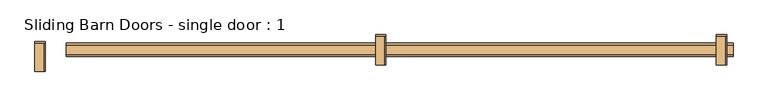
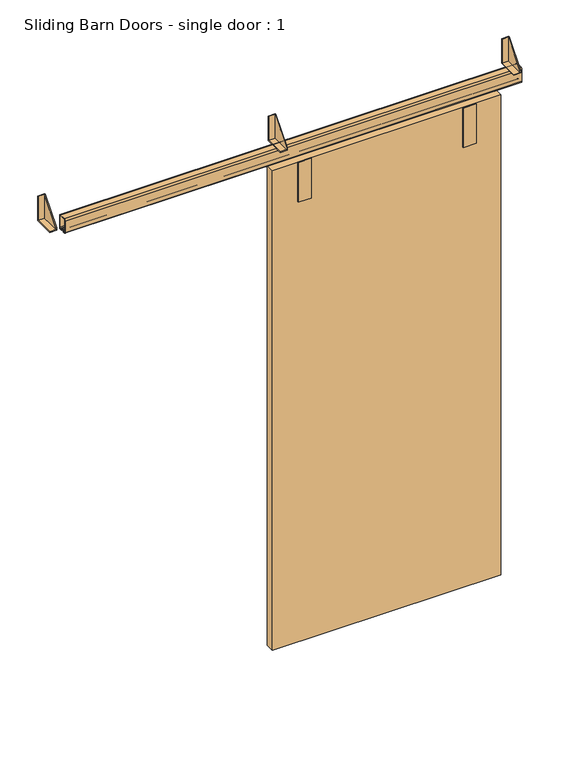
"""IFC4 building model written with IfcOpenShell, lengths in millimetres: door geometry, Sliding Barn Doors - single door : 1."""

from ifc_helpers import new_model, si_unit, point, frame, frame_2d, origin, place, context, project, spatial, polyline, circle_curve, trimmed, segment, composite_curve, outline, extrude, source, transform, mapped, element, save


def sliding_barn_doors_single_door_1_9618ed7f(model_context):
    return source(origin(), model_context, "Body", "SweptSolid", [
        extrude(outline(polyline([(-158.75, 2152.65), (-79.375, 2247.773), (-79.375, 2146.3), (-158.75, 2146.3), (-158.75, 2152.65)])), frame((-1418.4808594, 0.0, 0.0), z_axis=(1.0, 0.0, 0.0), x_axis=(0.0, 1.0, 0.0)), (0.0, 0.0, 1.0), 3.175),
        extrude(outline(polyline([(-76.2, 2143.125), (-158.75, 2143.125), (-158.75, 2146.3), (-79.375, 2146.3), (-79.375, 2247.773), (-76.2, 2247.773), (-76.2, 2143.125)])), frame((-1443.7816406, 0.0, 0.0), z_axis=(1.0, 0.0, 0.0), x_axis=(0.0, 1.0, 0.0)), (0.0, 0.0, 1.0), 28.4757812),
        extrude(outline(polyline([(-139.7, 2152.65), (-60.325, 2247.773), (-60.325, 2146.3), (-139.7, 2146.3), (-139.7, 2152.65)])), frame((-484.2371094, 0.0, 0.0), z_axis=(1.0, 0.0, 0.0), x_axis=(0.0, 1.0, 0.0)), (0.0, 0.0, 1.0), 3.175),
        extrude(outline(polyline([(-57.15, 2143.125), (-139.7, 2143.125), (-139.7, 2146.3), (-60.325, 2146.3), (-60.325, 2247.773), (-57.15, 2247.773), (-57.15, 2143.125)])), frame((-509.5378906, 0.0, 0.0), z_axis=(1.0, 0.0, 0.0), x_axis=(0.0, 1.0, 0.0)), (0.0, 0.0, 1.0), 28.4757813),
        extrude(outline(polyline([(-139.7, 2152.65), (-60.325, 2247.773), (-60.325, 2146.3), (-139.7, 2146.3), (-139.7, 2152.65)])), frame((450.0066406, 0.0, 0.0), z_axis=(1.0, 0.0, 0.0), x_axis=(0.0, 1.0, 0.0)), (0.0, 0.0, 1.0), 3.175),
        extrude(outline(polyline([(-57.15, 2143.125), (-139.7, 2143.125), (-139.7, 2146.3), (-60.325, 2146.3), (-60.325, 2247.773), (-57.15, 2247.773), (-57.15, 2143.125)])), frame((424.7058594, 0.0, 0.0), z_axis=(1.0, 0.0, 0.0), x_axis=(0.0, 1.0, 0.0)), (0.0, 0.0, 1.0), 28.4757813),
        extrude(outline(polyline([(-424.91025, -117.475), (-424.91025, -114.3), (-373.60225, -114.3), (-373.60225, -117.475), (-424.91025, -117.475)])), frame((0.0, 0.0, 1889.252), z_axis=(0.0, 0.0, 1.0), x_axis=(1.0, 0.0, 0.0)), (0.0, 0.0, 1.0), 168.148),
        extrude(outline(polyline([(235.48975, -117.475), (235.48975, -114.3), (286.79775, -114.3), (286.79775, -117.475), (235.48975, -117.475)])), frame((0.0, 0.0, 1889.252), z_axis=(0.0, 0.0, 1.0), x_axis=(1.0, 0.0, 0.0)), (0.0, 0.0, 1.0), 168.148),
        extrude(outline(polyline([(-526.25625, -114.3), (-526.25625, -79.375), (388.14375, -79.375), (388.14375, -114.3), (-526.25625, -114.3)])), frame((0.0, 0.0, 25.4), z_axis=(0.0, 0.0, 1.0), x_axis=(1.0, 0.0, 0.0)), (0.0, 0.0, 1.0), 2032.0),
        extrude(outline(composite_curve([segment(trimmed(circle_curve(frame_2d((-85.725, 2136.775)), 6.35), [point((-85.725, 2143.125))], [point((-79.375, 2136.775))], False, "CARTESIAN"), True, "CONTINUOUS"), segment(polyline([(-79.375, 2136.775), (-79.375, 2088.515)]), True, "CONTINUOUS"), segment(trimmed(circle_curve(frame_2d((-85.725, 2088.515)), 6.35), [point((-79.375, 2088.515))], [point((-85.725, 2082.165))], False, "CARTESIAN"), True, "CONTINUOUS"), segment(polyline([(-85.725, 2082.165), (-91.1336853, 2082.165)]), True, "CONTINUOUS"), segment(trimmed(circle_curve(frame_2d((-91.1336853, 2083.7525)), 1.5875), [point((-91.1336853, 2082.165))], [point((-92.6920184, 2083.4495907))], False, "CARTESIAN"), True, "CONTINUOUS"), segment(polyline([(-92.6920184, 2083.4495907), (-94.1175341, 2090.7832331), (-92.6013971, 2090.7832331), (-91.2154749, 2083.6532812), (-85.725, 2083.6532812)]), True, "CONTINUOUS"), segment(trimmed(circle_curve(frame_2d((-85.725, 2088.515)), 4.8617187), [point((-85.725, 2083.6532812))], [point((-80.8632813, 2088.515))], True, "CARTESIAN"), True, "CONTINUOUS"), segment(polyline([(-80.8632813, 2088.515), (-80.8632813, 2136.775)]), True, "CONTINUOUS"), segment(trimmed(circle_curve(frame_2d((-85.725, 2136.775)), 4.8617187), [point((-80.8632813, 2136.775))], [point((-85.725, 2141.6367187))], True, "CARTESIAN"), True, "CONTINUOUS"), segment(polyline([(-85.725, 2141.6367187), (-111.252, 2141.6367187)]), True, "CONTINUOUS"), segment(trimmed(circle_curve(frame_2d((-111.252, 2136.775)), 4.8617187), [point((-111.252, 2141.6367187))], [point((-116.1137188, 2136.775))], True, "CARTESIAN"), True, "CONTINUOUS"), segment(polyline([(-116.1137188, 2136.775), (-116.1137188, 2088.515)]), True, "CONTINUOUS"), segment(trimmed(circle_curve(frame_2d((-111.252, 2088.515)), 4.8617187), [point((-116.1137188, 2088.515))], [point((-111.252, 2083.6532812))], True, "CARTESIAN"), True, "CONTINUOUS"), segment(polyline([(-111.252, 2083.6532812), (-105.7615251, 2083.6532812), (-104.3756029, 2090.7832331), (-102.8594659, 2090.7832331), (-104.2849816, 2083.4495907)]), True, "CONTINUOUS"), segment(trimmed(circle_curve(frame_2d((-105.8433147, 2083.7525)), 1.5875), [point((-104.2849816, 2083.4495907))], [point((-105.8433147, 2082.165))], False, "CARTESIAN"), True, "CONTINUOUS"), segment(polyline([(-105.8433147, 2082.165), (-111.252, 2082.165)]), True, "CONTINUOUS"), segment(trimmed(circle_curve(frame_2d((-111.252, 2088.515)), 6.35), [point((-111.252, 2082.165))], [point((-117.602, 2088.515))], False, "CARTESIAN"), True, "CONTINUOUS"), segment(polyline([(-117.602, 2088.515), (-117.602, 2136.775)]), True, "CONTINUOUS"), segment(trimmed(circle_curve(frame_2d((-111.252, 2136.775)), 6.35), [point((-117.602, 2136.775))], [point((-111.252, 2143.125))], False, "CARTESIAN"), True, "CONTINUOUS"), segment(polyline([(-111.252, 2143.125), (-85.725, 2143.125)]), True, "CONTINUOUS")], self_intersect=False)), frame((-1358.10625, 0.0, 0.0), z_axis=(1.0, 0.0, 0.0), x_axis=(0.0, 1.0, 0.0)), (0.0, 0.0, 1.0), 1828.8),
    ])


if __name__ == "__main__":
    model = new_model("IFC4")
    model_context = context("Model", 3, world=origin())
    ifc_project = project(units=[si_unit("LENGTHUNIT", "METRE", prefix="MILLI")], contexts=[model_context])
    site = spatial("IfcSite", under=ifc_project)
    building = spatial("IfcBuilding", under=site)
    placement = place(None, origin())
    sliding_barn_doors_single_door_1_shape = sliding_barn_doors_single_door_1_9618ed7f(model_context)
    element("IfcDoor", 1, ObjectType="Sliding Barn Doors - single door : 1", at=placement, inside=building, context=model_context, shape_type="MappedRepresentation", body=[
        mapped(sliding_barn_doors_single_door_1_shape, transform((0.0, 0.0, 0.0), x_axis=(1.0, 0.0, 0.0), y_axis=(0.0, 1.0, 0.0), z_axis=(0.0, 0.0, 1.0))),
    ])
    save(model, "model.ifc")

# Revit data of these elements
# Type "Sliding Barn Doors - single door : 1"
#   Type Mark = "61"
#   OD_DS_Door_Material = "T.B.D."
#   OD_DS_Door_Type = "SLIDER"
#   OD_DS_Lockset = "-"
#   Analytic Construction = "<None>"
#   rail_overlap_left = 0' - 5 1/4"
#   rail_length = 6' - 0"
#   overlap_left = 0' - 2"
#   overlap = 0' - 0"
#   bracket_right = 3' - 7"
#   bracket_left = 0' - 4"
#   Thickness = 0' - 1 3/8"
#   Panel Width = 3' - 0"
#   Panel Height = 6' - 8"
#   Gap 2 = 0' - 0 1/2"
#   Gap 1 = 0' - 0 7/8"
#   Frame Projection Ext. = 0' - 1"
#   Frame Projection Int. = 0' - 1"
#   Frame Width = 0' - 3"
#   Height = 6' - 4"
#   Width = 2' - 2 9/16"
#   Bracket_offset = 0' - 5"
#   Door_4 = no
#   Door_3 = no
#   Hardware Material = Metal - Aluminum
#   Door Material = Closet_1
#   Function = (empty or 0)
#   Wall Closure = (empty or 0)
# Element 1 (IfcDoor, "Sliding Barn Doors - single door : 1")
#   Materials on its faces: "Metal - Aluminum", "Closet_1"
# Materials
#   "Metal - Aluminum": class "Metal", colour RGB 247 247 247, transparency 0
#   "Closet_1": class "Paint", colour RGB 200 194 183, transparency 0, Cost = 0
